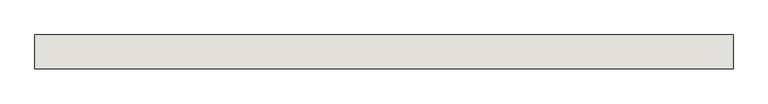
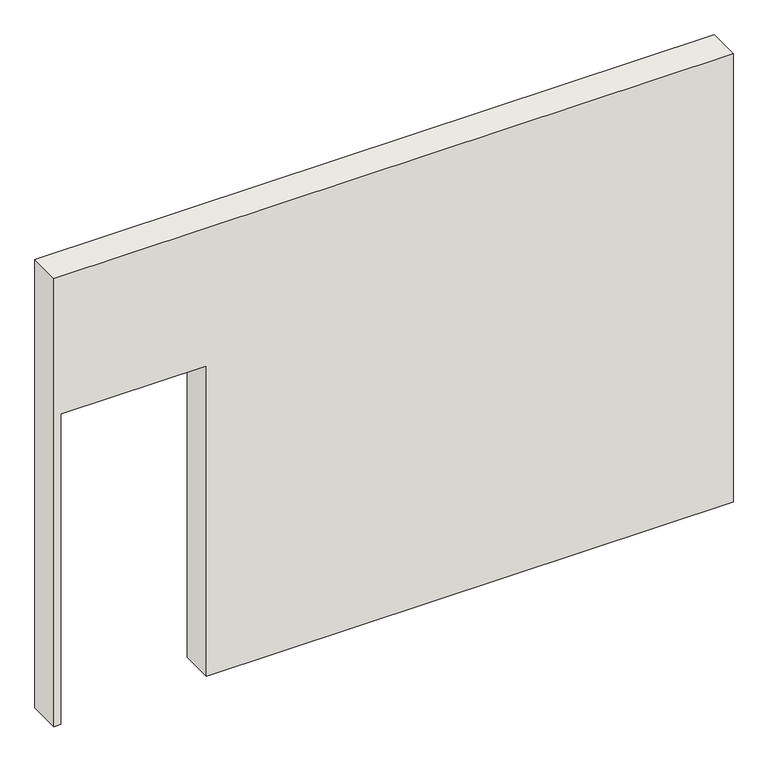
"""IFC4 building model written with IfcOpenShell, lengths in millimetres: wall geometry, Holzwand."""

import ifcopenshell
import ifcopenshell.guid

model = None  # the IFC model being written
_history = None  # IfcOwnerHistory: only IFC2X3 demands one
_inside = {}  # id of a spatial element -> (the spatial element, [elements in it])
_under = {}  # id of a project, library or spatial element -> (it, [spatial elements below it])
_declared = {}  # id of a project -> (the project, [libraries it declares])
_typed = {}  # id of a type object -> (the type object, [elements of that type])
_made_of = {}  # id of a material, layer set ... -> (it, [elements and type objects made of it])


def new_model(schema):
    """Start an empty IFC model of exactly this schema.

    Asked for "IFC4X3", IfcOpenShell would pick the latest addendum, in which some entities
    have other attributes; the version numbers below select the first issue.
    IFC2X3 requires an IfcOwnerHistory on every rooted entity: one is made here for all.
    """
    global model, _history
    if schema == "IFC4X3":
        model = ifcopenshell.file(schema_version=(4, 3, 0, 0))
    else:
        model = ifcopenshell.file(schema=schema)
    _inside.clear()
    _under.clear()
    _declared.clear()
    _typed.clear()
    _made_of.clear()
    _history = None
    if model.schema == "IFC2X3":
        org = make("IfcOrganization", Name="unknown")
        user = make(
            "IfcPersonAndOrganization",
            ThePerson=make("IfcPerson", FamilyName="unknown"),
            TheOrganization=org,
        )
        app = make(
            "IfcApplication",
            ApplicationDeveloper=org,
            Version="unknown",
            ApplicationFullName="unknown",
            ApplicationIdentifier="unknown",
        )
        _history = make(
            "IfcOwnerHistory",
            OwningUser=user,
            OwningApplication=app,
            ChangeAction="ADDED",
            CreationDate=0,
        )
    return model


def make(cls, **values):
    """One entity of the class cls with the attributes given. An attribute that is None is left unset."""
    return model.create_entity(
        cls, **{name: value for name, value in values.items() if value is not None}
    )


def rooted(cls, **values):
    """An entity with a GlobalId (a new one), such as an element, a storey or a relation."""
    return make(cls, GlobalId=ifcopenshell.guid.new(), OwnerHistory=_history, **values)


def si_unit(unit_type, name, prefix=None):
    """IfcSIUnit, for example si_unit("LENGTHUNIT", "METRE", prefix="MILLI")."""
    return make("IfcSIUnit", UnitType=unit_type, Prefix=prefix, Name=name)


def assignment(units):
    """IfcUnitAssignment: the units of a project."""
    return None if units is None else make("IfcUnitAssignment", Units=units)


def point(xyz):
    """IfcCartesianPoint."""
    return None if xyz is None else make("IfcCartesianPoint", Coordinates=xyz)


def direction(xyz):
    """IfcDirection."""
    return None if xyz is None else make("IfcDirection", DirectionRatios=xyz)


def frame(location, z_axis=None, x_axis=None):
    """IfcAxis2Placement3D, a coordinate frame: its origin and axes. An axis left out is left unset."""
    return make(
        "IfcAxis2Placement3D",
        Location=point(location),
        Axis=direction(z_axis),
        RefDirection=direction(x_axis),
    )


def origin():
    """The frame at (0, 0, 0) with its axes left unset."""
    return frame((0.0, 0.0, 0.0))


def place(relative_to, where):
    """IfcLocalPlacement: puts the frame where relative to a parent placement (None: the world)."""
    return make(
        "IfcLocalPlacement", PlacementRelTo=relative_to, RelativePlacement=where
    )


def context(
    kind, dimensions, precision=None, world=None, true_north=None, identifier=None
):
    """IfcGeometricRepresentationContext, for example the 3D "Model" context."""
    return make(
        "IfcGeometricRepresentationContext",
        ContextIdentifier=identifier,
        ContextType=kind,
        CoordinateSpaceDimension=dimensions,
        Precision=precision,
        WorldCoordinateSystem=world,
        TrueNorth=true_north,
    )


def project(units=None, contexts=None):
    """IfcProject with its units and contexts."""
    return rooted(
        "IfcProject",
        Name="project",
        RepresentationContexts=contexts,
        UnitsInContext=assignment(units),
    )


def spatial(cls, under=None, at=None, **own):
    """A site, building, storey or space (cls), placed at a placement, below another one or the project."""
    s = rooted(cls, ObjectPlacement=at, **own)
    if under is not None:
        _under.setdefault(under.id(), (under, []))[1].append(s)
    return s


def polyline(points):
    """IfcPolyline through the points."""
    return make("IfcPolyline", Points=[point(p) for p in points])


def outline(outer, holes=None, kind="AREA"):
    """IfcArbitraryClosedProfileDef: a profile drawn as a closed curve; with holes, ...WithVoids."""
    if holes is None:
        return make("IfcArbitraryClosedProfileDef", ProfileType=kind, OuterCurve=outer)
    return make(
        "IfcArbitraryProfileDefWithVoids",
        ProfileType=kind,
        OuterCurve=outer,
        InnerCurves=holes,
    )


def extrude(swept, where, along, depth):
    """IfcExtrudedAreaSolid: the profile swept, set in the frame where, extruded along a direction by depth."""
    return make(
        "IfcExtrudedAreaSolid",
        SweptArea=swept,
        Position=where,
        ExtrudedDirection=direction(along),
        Depth=depth,
    )


def shape(context_of_items, identifier, shape_type, items):
    """IfcShapeRepresentation: the items that make up one representation, for example the "Body"."""
    return make(
        "IfcShapeRepresentation",
        ContextOfItems=context_of_items,
        RepresentationIdentifier=identifier,
        RepresentationType=shape_type,
        Items=items,
    )


def source(mapping_origin, context_of_items, identifier, shape_type, items):
    """IfcRepresentationMap: a shape defined once, which mapped items show again and again."""
    return make(
        "IfcRepresentationMap",
        MappingOrigin=mapping_origin,
        MappedRepresentation=shape(context_of_items, identifier, shape_type, items),
    )


def transform(
    local_origin,
    x_axis=None,
    y_axis=None,
    z_axis=None,
    scale=None,
    scale2=None,
    scale3=None,
    uniform=True,
):
    """IfcCartesianTransformationOperator3D, or its non-uniform kind. x_axis, y_axis, z_axis: its Axis1, 2, 3."""
    if uniform:
        return make(
            "IfcCartesianTransformationOperator3D",
            Axis1=direction(x_axis),
            Axis2=direction(y_axis),
            LocalOrigin=point(local_origin),
            Scale=scale,
            Axis3=direction(z_axis),
        )
    return make(
        "IfcCartesianTransformationOperator3DnonUniform",
        Axis1=direction(x_axis),
        Axis2=direction(y_axis),
        LocalOrigin=point(local_origin),
        Scale=scale,
        Axis3=direction(z_axis),
        Scale2=scale2,
        Scale3=scale3,
    )


def mapped(mapping_source, mapping_target):
    """IfcMappedItem: shows the shape of a source again, moved by a transform."""
    return make(
        "IfcMappedItem", MappingSource=mapping_source, MappingTarget=mapping_target
    )


def made_of(thing, what):
    """Note that an element or type object is made of a material, layer set ...; save() writes the relation."""
    if what is not None:
        _made_of.setdefault(what.id(), (what, []))[1].append(thing)
    return thing


def element(
    cls,
    number,
    at=None,
    inside=None,
    cuts=None,
    type_object=None,
    material=None,
    context=None,
    identifier="Body",
    shape_type=None,
    held_by="IfcProductDefinitionShape",
    body=None,
    shapes=None,
    **own,
):
    """One element of the class cls, such as IfcWall. Its Tag is "e" and its number.

    at: its placement. inside: the storey or other place that contains it. cuts: it is an
    opening in that element (IfcRelVoidsElement). A single representation is given by context,
    identifier, shape_type and body (its items); several are given by shapes. held_by: the class
    of the entity that holds the representations. save() writes the other relations.
    """
    e = rooted(cls, Tag="e%d" % number, ObjectPlacement=at, **own)
    if body is not None:
        shapes = [shape(context, identifier, shape_type, body)]
    if shapes is not None:
        e.Representation = make(held_by, Representations=shapes)
    if inside is not None:
        _inside.setdefault(inside.id(), (inside, []))[1].append(e)
    if cuts is not None:
        rooted(
            "IfcRelVoidsElement", RelatingBuildingElement=cuts, RelatedOpeningElement=e
        )
    if type_object is not None:
        _typed.setdefault(type_object.id(), (type_object, []))[1].append(e)
    return made_of(e, material)


def aggregate(whole, parts):
    """IfcRelAggregates: a whole, such as a stair, and the parts it consists of."""
    return rooted("IfcRelAggregates", RelatingObject=whole, RelatedObjects=parts)


def save(model, path):
    """Write the relations noted so far, then the file.

    IfcRelAggregates (storeys below a building ...), IfcRelContainedInSpatialStructure (elements
    in a storey), IfcRelDefinesByType, IfcRelAssociatesMaterial and IfcRelDeclares: one each for
    every whole, place, type object, material and project.
    """
    for whole, parts in _under.values():
        aggregate(whole, parts)
    for where, things in _inside.values():
        rooted(
            "IfcRelContainedInSpatialStructure",
            RelatedElements=things,
            RelatingStructure=where,
        )
    for kind, things in _typed.values():
        rooted("IfcRelDefinesByType", RelatedObjects=things, RelatingType=kind)
    for what, things in _made_of.values():
        rooted("IfcRelAssociatesMaterial", RelatedObjects=things, RelatingMaterial=what)
    for by, libraries in _declared.values():
        rooted("IfcRelDeclares", RelatingContext=by, RelatedDefinitions=libraries)
    model.write(path)


def wall_c8f5c598(model_context):
    return source(origin(), model_context, "Body", "SweptSolid", [
        extrude(outline(polyline([(1995.0, 925.9795824), (0.0, 925.9795824), (0.0, 4125.9795824), (2880.0, 4125.9795824), (2880.0, 0.0), (0.0, 0.0), (0.0, 40.9795824), (1995.0, 40.9795824), (1995.0, 925.9795824)])), frame((0.0, 0.0, 0.0), z_axis=(0.0, 1.0, 0.0), x_axis=(0.0, 0.0, 1.0)), (0.0, 0.0, 1.0), 200.0),
    ])


if __name__ == "__main__":
    model = new_model("IFC4")
    model_context = context("Model", 3, world=origin())
    ifc_project = project(units=[si_unit("LENGTHUNIT", "METRE", prefix="MILLI")], contexts=[model_context])
    site = spatial("IfcSite", under=ifc_project)
    building = spatial("IfcBuilding", under=site)
    placement = place(None, origin())
    wall_shape = wall_c8f5c598(model_context)
    element("IfcWall", 1, ObjectType="Holzwand", at=placement, inside=building, context=model_context, shape_type="MappedRepresentation", body=[
        mapped(wall_shape, transform((0.0, 0.0, 0.0), x_axis=(1.0, 0.0, 0.0), y_axis=(0.0, 1.0, 0.0), z_axis=(0.0, 0.0, 1.0))),
    ])
    save(model, "model.ifc")

# Revit data of these elements
# Element 1 (IfcWall, "Holzwand")
#   Materials on its faces: "holzschalung"
# Materials
#   "holzschalung": class "Unassigned", colour RGB 128 128 128, transparency 0
